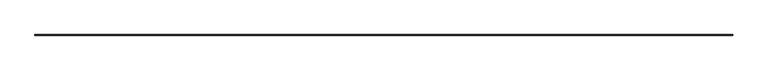
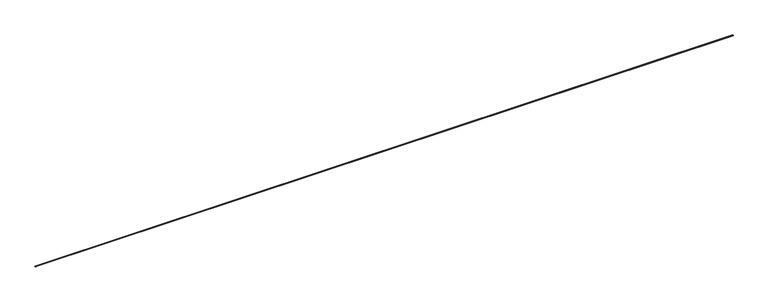
"""IFC4 building model written with IfcOpenShell, lengths in millimetres: proxy geometry, Inner panel:Inner panel:1:Inner panel:1 : Inner panel:Inner panel:300324:2:Inner panel:1:Inner panel:1 : Inner panel:Inner panel:300324:2 : Inner panel:Inner panel:1:Inner panel:1 : Inner panel:Inner panel:300324:300043:39 : Inner panel:Inner panel:1:Inner panel:1 : Inner panel:Inner panel:300324:2:Inner panel:1:Inner panel:1 : Inner panel:Inner panel:300324:2 : Inner panel:Inner panel:1:Inner panel:1 : Inner panel:Inner panel:300324:300043:308120."""

from ifc_helpers import new_model, si_unit, frame, origin, place, context, project, spatial, polyline, outline, extrude, source, transform, mapped, element, save


def generic_models_35238bca(model_context):
    return source(origin(), model_context, "Body", "SweptSolid", [
        extrude(outline(polyline([(-568088.0451322, 8769.6710731), (-568089.5651675, 8806.1519194), (-568132.4433237, 8804.3653295), (-568130.9232885, 8767.8844832), (-568147.5976955, 8767.1897163), (-568147.754936, 8770.9634892), (-568146.1660586, 8770.9634892), (-568146.0776602, 8768.8419285), (-568132.5755007, 8769.4045185), (-568134.095536, 8805.8853648), (-568088.0451322, 8807.8041316), (-568086.525097, 8771.3232853), (-568073.0229375, 8771.8858753), (-568073.1140895, 8774.0735244), (-568071.5252121, 8774.0735244), (-568071.3707252, 8770.36584), (-568088.0451322, 8769.6710731)])), frame((579104.5117239, 0.0, 0.0), z_axis=(1.0, 0.0, 0.0), x_axis=(0.0, 1.0, 0.0)), (0.0, 0.0, 1.0), 88442.8),
    ])


if __name__ == "__main__":
    model = new_model("IFC4")
    model_context = context("Model", 3, world=origin())
    ifc_project = project(units=[si_unit("LENGTHUNIT", "METRE", prefix="MILLI")], contexts=[model_context])
    site = spatial("IfcSite", under=ifc_project)
    building = spatial("IfcBuilding", under=site)
    placement = place(None, origin())
    generic_models_shape = generic_models_35238bca(model_context)
    element("IfcBuildingElementProxy", 1, Name="Inner panel:Inner panel:1:Inner panel:1 : Inner panel:Inner panel:300324:2:Inner panel:1:Inner panel:1 : Inner panel:Inner panel:300324:2 : Inner panel:Inner panel:1:Inner panel:1 : Inner panel:Inner panel:300324:300043:39 : Inner panel:Inner panel:1:Inner panel:1 : Inner panel:Inner panel:300324:2:Inner panel:1:Inner panel:1 : Inner panel:Inner panel:300324:2 : Inner panel:Inner panel:1:Inner panel:1 : Inner panel:Inner panel:300324:300043:308120", ObjectType="Inner panel:Inner panel:1:Inner panel:1 : Inner panel:Inner panel:300324:2:Inner panel:1:Inner panel:1 : Inner panel:Inner panel:300324:2 : Inner panel:Inner panel:1:Inner panel:1 : Inner panel:Inner panel:300324:300043:39 : Inner panel:Inner panel:1:Inner panel:1 : Inner panel:Inner panel:300324:2:Inner panel:1:Inner panel:1 : Inner panel:Inner panel:300324:2 : Inner panel:Inner panel:1:Inner panel:1 : Inner panel:Inner panel:300324:300043:308120", at=placement, inside=building, context=model_context, shape_type="MappedRepresentation", body=[
        mapped(generic_models_shape, transform((0.0, 0.0, 0.0), x_axis=(1.0, 0.0, 0.0), y_axis=(0.0, 1.0, 0.0), z_axis=(0.0, 0.0, 1.0))),
    ])
    save(model, "model.ifc")

# Revit data of these elements
# Type "Inner panel:Inner panel:1:Inner panel:1 : Inner panel:Inner panel:300324:2:Inner panel:1:Inner panel:1 : Inner panel:Inner panel:300324:2 : Inner panel:Inner panel:1:Inner panel:1 : Inner panel:Inner panel:300324:300043:39 : Inner panel:Inner panel:1:Inner panel:1 : Inner panel:Inner panel:300324:2:Inner panel:1:Inner panel:1 : Inner panel:Inner panel:300324:2 : Inner panel:Inner panel:1:Inner panel:1 : Inner panel:Inner panel:300324:300043:308120"
#   NameOverride = "Inner panel:Inner panel:1:Inner panel:1 : Inner panel:Inner panel:300324:2:Inner panel:1:Inner panel:1 : Inner panel:Inner panel:300324:2 : Inner panel:Inner panel:1:Inner panel:1 : Inner panel:Inner panel:300324:300043:308120"
#   ObjectTypeOverride = "Inner panel:1:Inner panel:1 : Inner panel:Inner panel:300324:2 : Inner panel:Inner panel:1:Inner panel:1 : Inner panel:Inner panel:300324:300043"
#   Reference = "Inner panel"
#   Tag = "308120"
# Element 1 (IfcBuildingElementProxy, "Inner panel:Inner panel:1:Inner panel:1 : Inner panel:Inner panel:300324:2:Inner panel:1:Inner panel:1 : Inner panel:Inner panel:300324:2 : Inner panel:Inner panel:1:Inner panel:1 : Inner panel:Inner panel:300324:300043:39 : Inner panel:Inner panel:1:Inner panel:1 : Inner panel:Inner panel:300324:2:Inner panel:1:Inner panel:1 : Inner panel:Inner panel:300324:2 : Inner panel:Inner panel:1:Inner panel:1 : Inner panel:Inner panel:300324:300043:308120")
#   Materials on its faces: "1 1/2\" HAT CHANNELS - SEE STRUCT. DWGs"
# Materials
#   "1 1/2\" HAT CHANNELS - SEE STRUCT. DWGs": class "Metal", colour RGB 189 187 185, transparency 0, Description = "Structural steel 50ksi", Cost = 0
